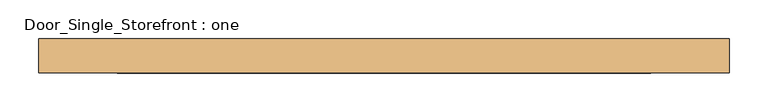
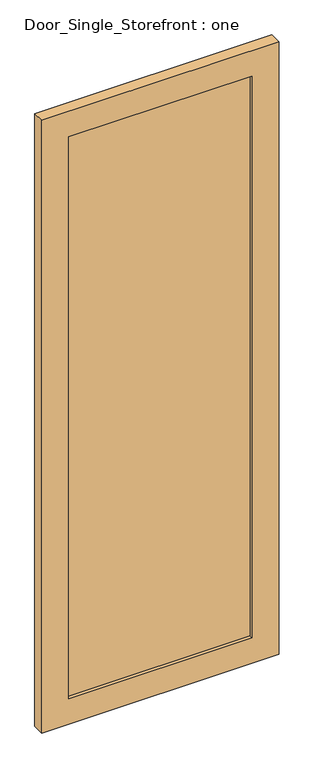
"""IFC4 building model written with IfcOpenShell, lengths in millimetres: door geometry, Door_Single_Storefront : one."""

from ifc_helpers import new_model, si_unit, frame, origin, place, context, project, spatial, polyline, outline, extrude, source, transform, mapped, element, save


def door_single_storefront_one_a0d18356(model_context):
    return source(origin(), model_context, "Body", "SweptSolid", [
        extrude(outline(polyline([(345.28125, -6.35), (-345.28125, -6.35), (-345.28125, 12.7), (345.28125, 12.7), (345.28125, -6.35)])), frame((0.0, 0.0, 101.6), z_axis=(0.0, 0.0, 1.0), x_axis=(1.0, 0.0, 0.0)), (0.0, 0.0, 1.0), 2235.2),
        extrude(outline(polyline([(2438.4, -446.88125), (0.0, -446.88125), (0.0, 446.88125), (2438.4, 446.88125), (2438.4, -446.88125)]), holes=[polyline([(101.6, 345.28125), (101.6, -345.28125), (2336.8, -345.28125), (2336.8, 345.28125), (101.6, 345.28125)])]), frame((0.0, -19.05, 0.0), z_axis=(0.0, 1.0, 0.0), x_axis=(0.0, 0.0, 1.0)), (0.0, 0.0, 1.0), 44.45),
    ])


if __name__ == "__main__":
    model = new_model("IFC4")
    model_context = context("Model", 3, world=origin())
    ifc_project = project(units=[si_unit("LENGTHUNIT", "METRE", prefix="MILLI")], contexts=[model_context])
    site = spatial("IfcSite", under=ifc_project)
    building = spatial("IfcBuilding", under=site)
    placement = place(None, origin())
    door_single_storefront_one_shape = door_single_storefront_one_a0d18356(model_context)
    element("IfcDoor", 1, ObjectType="Door_Single_Storefront : one", at=placement, inside=building, context=model_context, shape_type="MappedRepresentation", body=[
        mapped(door_single_storefront_one_shape, transform((0.0, 0.0, 0.0), x_axis=(1.0, 0.0, 0.0), y_axis=(0.0, 1.0, 0.0), z_axis=(0.0, 0.0, 1.0))),
    ])
    save(model, "model.ifc")

# Revit data of these elements
# Type "Door_Single_Storefront : one"
#   Type Mark = "27"
#   Analytic Construction = "<None>"
#   Stile_Width = 0' - 4"
#   Door_Thickness = 0' - 1 3/4"
#   Door_Offset = 0' - 1"
#   Glass_Material = Glass
#   Frame_Material = Aluminum
#   Function = (empty or 0)
# Element 1 (IfcDoor, "Door_Single_Storefront : one")
#   Materials on its faces: "Aluminum", "Glass"
# Materials
#   "Glass": class "Glass", colour RGB 142 168 196, transparency 0.75, Description = "Soda Lime Glass", Cost = 0
#   "Aluminum": class "Metal", colour RGB 226 226 226, transparency 0, Description = "Aluminum 6061", Cost = 0
